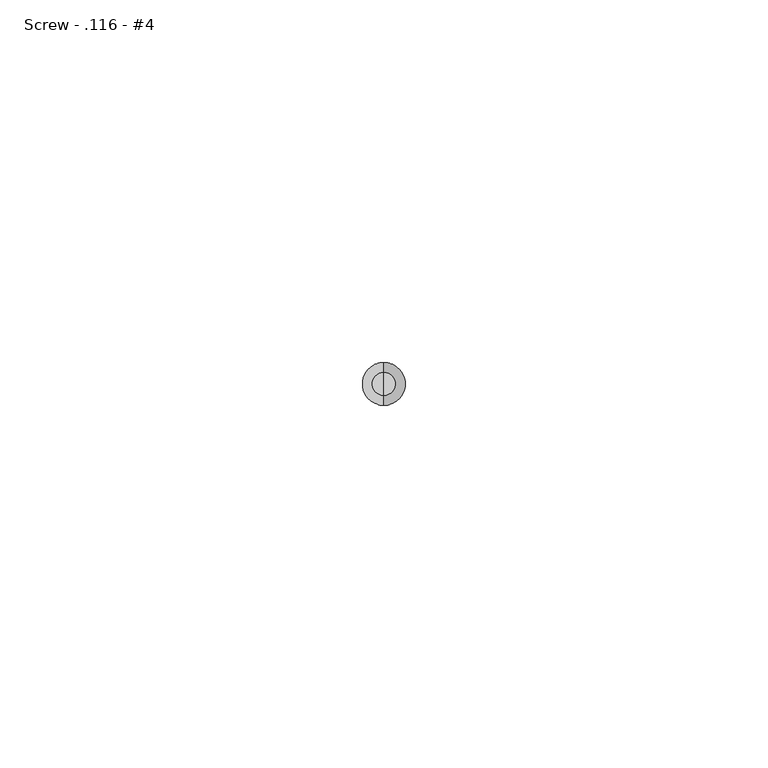
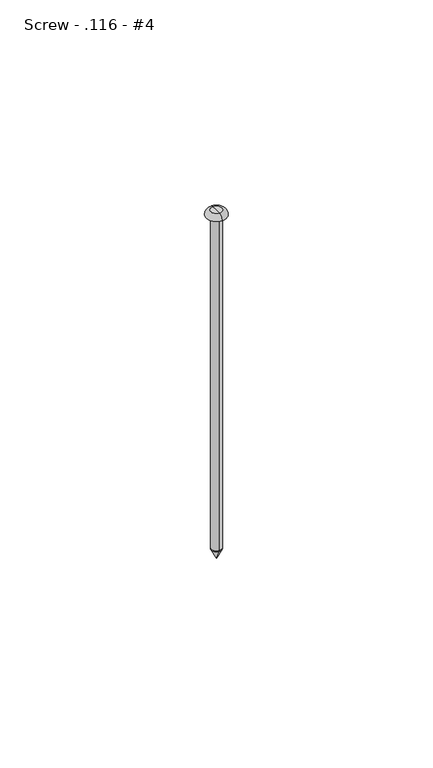
"""IFC4 building model written with IfcOpenShell, lengths in millimetres: fastener geometry, 060523 - W_P_C - Fastenings - Generic : Screw - .116 - #4."""

from ifc_helpers import new_model, si_unit, point, frame, origin, origin_2d, place, context, project, spatial, polyline, circle_curve, ellipse_curve, trimmed, segment, composite_curve, outline, extrude, source, transform, mapped, element, save
from ifc_brep_helpers import plane_surface, revolved_surface, advanced_brep


def screw_116_4_5c189c7d(model_context):
    return source(origin(), model_context, "Body", "SolidModel", [
        advanced_brep(
        [(0.0, -1.4732, -101.6), (0.0, 1.4732, -101.6), (0.0, 0.0, -101.6), (0.0, 0.0, -104.5464)],
        [
            (0, 1, circle_curve(frame((0.0, 0.0, -101.6), z_axis=(0.0, 0.0, 1.0), x_axis=(0.0, 1.0, 0.0)), 1.4732)),
            (1, 2),
            (2, 0),
            (1, 0, circle_curve(frame((0.0, 0.0, -101.6), z_axis=(0.0, 0.0, 1.0), x_axis=(0.0, 1.0, 0.0)), 1.4732)),
            (3, 1),
            (0, 3),
        ],
        [
            plane_surface(frame((0.0, 0.0, -101.6), z_axis=(0.0, 0.0, 1.0), x_axis=(0.0, 1.0, 0.0))),
            revolved_surface(polyline([(0.0, 1.4732, -101.6), (0.0, 0.0, -104.5464)]), (0.0, 0.0, -103.0840259), (0.0, 0.0, -1.0)),
        ],
        [
            (0, [[1, 2, 3]]),
            (0, [[4, -3, -2]]),
            (1, [[5, -1, 6]]),
            (1, [[-6, -4, -5]]),
        ],
    ),
        advanced_brep(
        [(0.0, 2.9464, 0.0), (0.0, -2.9464, 0.0), (0.0, 0.0, 0.0), (0.0, 0.0, 1.4732), (0.0, -1.5875, 1.4732), (0.0, 1.5875, 1.4732)],
        [
            (0, 1, circle_curve(frame((0.0, 0.0, 0.0), z_axis=(0.0, 0.0, -1.0), x_axis=(0.0, -1.0, 0.0)), 2.9464)),
            (1, 2),
            (2, 0),
            (1, 0, circle_curve(frame((0.0, 0.0, 0.0), z_axis=(0.0, 0.0, -1.0), x_axis=(0.0, -1.0, 0.0)), 2.9464)),
            (3, 4),
            (4, 5, circle_curve(frame((0.0, 0.0, 1.4732), z_axis=(0.0, 0.0, 1.0), x_axis=(0.0, -1.0, 0.0)), 1.5875)),
            (5, 3),
            (5, 4, circle_curve(frame((0.0, 0.0, 1.4732), z_axis=(0.0, 0.0, 1.0), x_axis=(0.0, -1.0, 0.0)), 1.5875)),
            (4, 1, circle_curve(frame((0.0, -1.5875, 0.1098659), z_axis=(1.0, 0.0, 0.0), x_axis=(0.0, -1.0, 0.0)), 1.3633341)),
            (0, 5, circle_curve(frame((0.0, 1.5875, 0.1098659), z_axis=(1.0, 0.0, 0.0), x_axis=(0.0, 1.0, 0.0)), 1.3633341)),
        ],
        [
            plane_surface(frame((0.0, 0.0, 0.0), z_axis=(0.0, 0.0, -1.0), x_axis=(0.0, -1.0, 0.0))),
            plane_surface(frame((0.0, 0.0, 1.4732), z_axis=(0.0, 0.0, 1.0), x_axis=(0.0, -1.0, 0.0))),
            revolved_surface(trimmed(ellipse_curve(frame((0.0, -1.5875, 0.1098659), z_axis=(-1.0, 0.0, 0.0), x_axis=(0.0, -1.0, 0.0)), 1.3633341, 1.3633341), [point((0.0, -2.9464, 0.0))], [point((0.0, -1.5875, 1.4732))], True, "CARTESIAN"), (0.0, 0.0, 1.4840259), (0.0, 0.0, 1.0)),
        ],
        [
            (0, [[1, 2, 3]]),
            (0, [[4, -3, -2]]),
            (1, [[5, 6, 7]]),
            (1, [[-7, 8, -5]]),
            (2, [[-6, 9, -1, 10]]),
            (2, [[-8, -10, -4, -9]]),
        ],
    ),
        extrude(outline(composite_curve([segment(trimmed(circle_curve(origin_2d(), 1.4732), [point((0.0, -1.4732))], [point((0.0, 1.4732))], False, "CARTESIAN"), True, "CONTINUOUS"), segment(trimmed(circle_curve(origin_2d(), 1.4732), [point((0.0, 1.4732))], [point((0.0, -1.4732))], False, "CARTESIAN"), True, "CONTINUOUS")], self_intersect=False)), frame((0.0, 0.0, -101.6), z_axis=(0.0, 0.0, 1.0), x_axis=(1.0, 0.0, 0.0)), (0.0, 0.0, 1.0), 101.6),
    ])


if __name__ == "__main__":
    model = new_model("IFC4")
    model_context = context("Model", 3, world=origin())
    ifc_project = project(units=[si_unit("LENGTHUNIT", "METRE", prefix="MILLI")], contexts=[model_context])
    site = spatial("IfcSite", under=ifc_project)
    building = spatial("IfcBuilding", under=site)
    placement = place(None, origin())
    screw_116_4_shape = screw_116_4_5c189c7d(model_context)
    element("IfcFastener", 1, ObjectType="060523 - W_P_C - Fastenings - Generic : Screw - .116 - #4", at=placement, inside=building, context=model_context, shape_type="MappedRepresentation", body=[
        mapped(screw_116_4_shape, transform((0.0, 0.0, 0.0), x_axis=(1.0, 0.0, 0.0), y_axis=(0.0, 1.0, 0.0), z_axis=(0.0, 0.0, 1.0))),
    ])
    save(model, "model.ifc")

# Revit data of these elements
# Type "060523 - W_P_C - Fastenings - Generic : Screw - .116 - #4"
#   Washer_Thickness = 0' - 0.00333"
#   Washer Radius = 0' - 0.068"
#   Washer Offset - Head = 0' - 0"
#   Washer Offset = 0' - 0"
#   Thickness_of_Substrate [instance default] = 0' - 1"
#   Side = 0' - 0 37/64"
#   Radius = 0' - 0.058"
#   Length [instance default] = 0' - 4"
#   Head Size = 0' - 1"
#   Head Radius = 0' - 0 1/2"
#   Head Height = 0' - 0.01"
#   Double Diameter = 0' - 0.232"
#   Diameter = 0' - 0.116"
#   Default Elevation = 4' - 0"
#   Washer_Nut_Visibility = no
#   Washer_Head_Visibility = no
#   Round_Head_Visibility = yes
#   Point Visibility = yes
#   Nut_Visibility = no
#   Hex_Head_Visiblilty = no
#   Washer Material = none
#   Bolt Material (Size) = AT SILL - FASTENER AT 24" O.C.
# Element 1 (IfcFastener, "060523 - W_P_C - Fastenings - Generic : Screw - .116 - #4")
#   Materials on its faces: "AT SILL - FASTENER AT 24\" O.C."
# Materials
#   "AT SILL - FASTENER AT 24\" O.C.": class "Generic", colour RGB 120 120 120, transparency 0, Cost = 0
